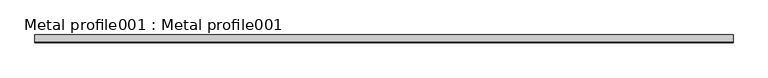
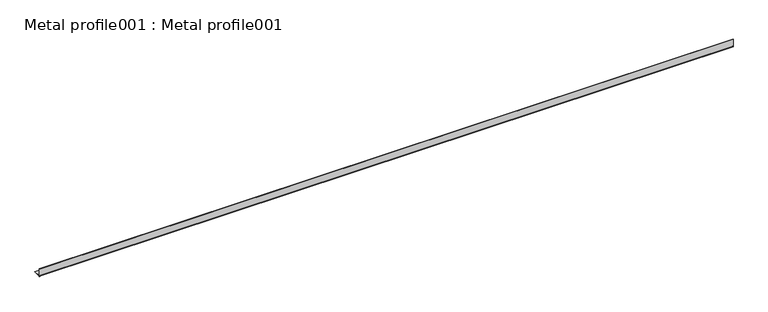
"""IFC4 building model written with IfcOpenShell, lengths in millimetres: proxy geometry, Metal profile001 : Metal profile001."""

from ifc_helpers import new_model, si_unit, point, frame, frame_2d, origin, place, context, project, spatial, polyline, circle_curve, trimmed, segment, composite_curve, outline, extrude, source, transform, mapped, element, save


def metal_profile001_metal_profile001_db72ebd8(model_context):
    return source(origin(), model_context, "Body", "SweptSolid", [
        extrude(outline(composite_curve([segment(polyline([(10196.5677938, 39423.8851145), (10196.5677938, 39402.7319306), (10217.7209778, 39402.7319306), (10217.7209778, 39401.4519306), (10196.8180681, 39401.4519306)]), True, "CONTINUOUS"), segment(trimmed(circle_curve(frame_2d((10195.9277938, 39402.0919306)), 1.0964434), [point((10196.8180681, 39401.4519306))], [point((10195.2877938, 39402.9822048))], False, "CARTESIAN"), True, "CONTINUOUS"), segment(polyline([(10195.2877938, 39402.9822048), (10195.2877938, 39423.8851145), (10196.5677938, 39423.8851145)]), True, "CONTINUOUS")], self_intersect=False)), frame((3694.2883192, 0.0, 0.0), z_axis=(1.0, 0.0, 0.0), x_axis=(0.0, 1.0, 0.0)), (0.0, 0.0, 1.0), 2000.0),
    ])


if __name__ == "__main__":
    model = new_model("IFC4")
    model_context = context("Model", 3, world=origin())
    ifc_project = project(units=[si_unit("LENGTHUNIT", "METRE", prefix="MILLI")], contexts=[model_context])
    site = spatial("IfcSite", under=ifc_project)
    building = spatial("IfcBuilding", under=site)
    placement = place(None, origin())
    metal_profile001_metal_profile001_shape = metal_profile001_metal_profile001_db72ebd8(model_context)
    element("IfcBuildingElementProxy", 1, Name="Metal profile001 : Metal profile001", ObjectType="Metal profile001 : Metal profile001", at=placement, inside=building, context=model_context, shape_type="MappedRepresentation", body=[
        mapped(metal_profile001_metal_profile001_shape, transform((0.0, 0.0, 0.0), x_axis=(1.0, 0.0, 0.0), y_axis=(0.0, 1.0, 0.0), z_axis=(0.0, 0.0, 1.0))),
    ])
    save(model, "model.ifc")

# Revit data of these elements
# Type "Metal profile001 : Metal profile001"
#   NameOverride = "Metal profile001"
# Element 1 (IfcBuildingElementProxy, "Metal profile001 : Metal profile001")
#   Materials on its faces: "CORNER BEAD"
# Materials
#   "CORNER BEAD": class "Unassigned", colour RGB 253 236 176, transparency 0, Cost = 0
